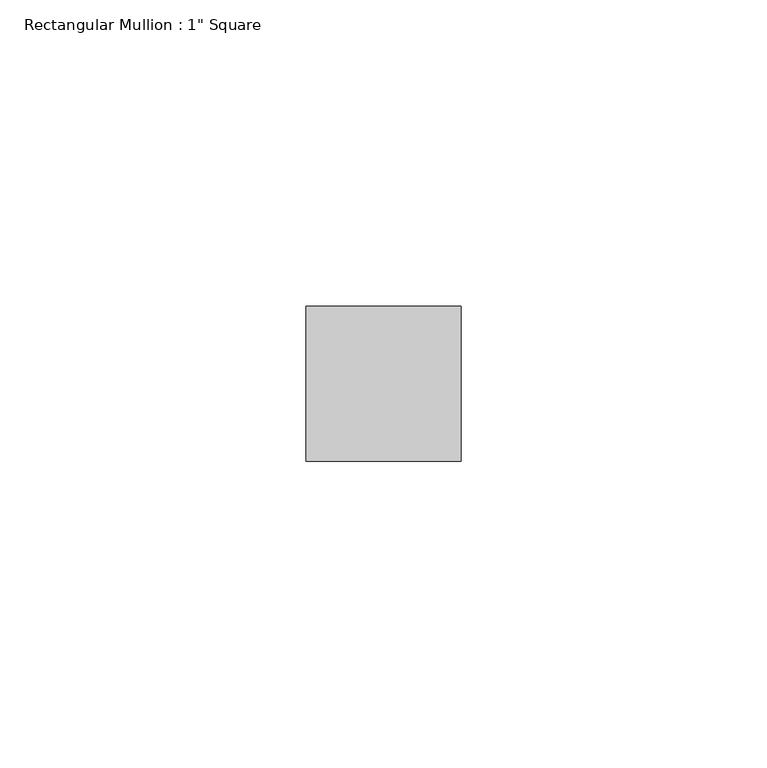
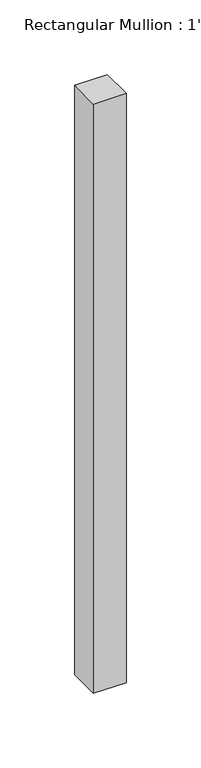
"""IFC4 building model written with IfcOpenShell, lengths in millimetres: member geometry."""

from ifc_helpers import new_model, si_unit, frame, origin, place, context, project, spatial, polyline, outline, extrude, source, transform, mapped, element, save


def member_6f1f35e1(model_context):
    return source(origin(), model_context, "Body", "SweptSolid", [
        extrude(outline(polyline([(0.0, 12.7), (0.0, -12.7), (-25.4, -12.7), (-25.4, 12.7), (0.0, 12.7)])), frame((0.0, 0.0, -482.6), z_axis=(0.0, 0.0, 1.0), x_axis=(1.0, 0.0, 0.0)), (0.0, 0.0, 1.0), 482.6),
    ])


if __name__ == "__main__":
    model = new_model("IFC4")
    model_context = context("Model", 3, world=origin())
    ifc_project = project(units=[si_unit("LENGTHUNIT", "METRE", prefix="MILLI")], contexts=[model_context])
    site = spatial("IfcSite", under=ifc_project)
    building = spatial("IfcBuilding", under=site)
    placement = place(None, origin())
    member_shape = member_6f1f35e1(model_context)
    element("IfcMember", 1, ObjectType="Rectangular Mullion : 1\" Square", at=placement, inside=building, context=model_context, shape_type="MappedRepresentation", body=[
        mapped(member_shape, transform((0.0, 0.0, 0.0), x_axis=(1.0, 0.0, 0.0), y_axis=(0.0, 1.0, 0.0), z_axis=(0.0, 0.0, 1.0))),
    ])
    save(model, "model.ifc")

# Revit data of these elements
# Type "Rectangular Mullion : 1\" Square"
#   built-in parameter 1007304 = 0.0833333 (stored number, unit not read)
#   built-in parameter 1007301 = 0.0416667 (stored number, unit not read)
#   built-in parameter 1007300 = 0.0416667 (stored number, unit not read)
# Element 1 (IfcMember, "Rectangular Mullion : 1\" Square")
#   Materials on its faces: "Metal - Aluminum"
# Materials
#   "Metal - Aluminum": class "Metal", colour RGB 247 247 247, transparency 0
